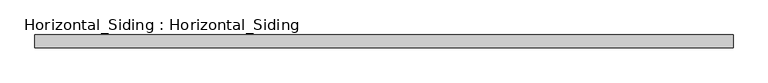
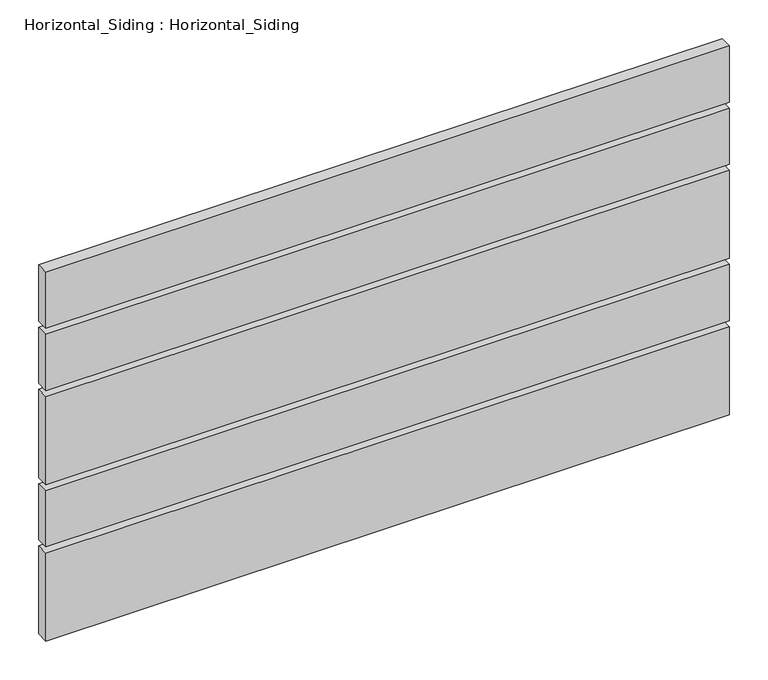
"""IFC4 building model written with IfcOpenShell, lengths in millimetres: plate geometry, Horizontal_Siding : Horizontal_Siding."""

from ifc_helpers import new_model, si_unit, frame, origin, place, context, project, spatial, polyline, outline, extrude, source, transform, mapped, element, save


def horizontal_siding_horizontal_siding_4d57135c(model_context):
    return source(origin(), model_context, "Body", "SweptSolid", [
        extrude(outline(polyline([(511.725524, -19.05), (-511.725524, -19.05), (-511.725524, 0.0), (511.725524, 0.0), (511.725524, -19.05)])), frame((0.0, 0.0, 9.525), z_axis=(0.0, 0.0, 1.0), x_axis=(1.0, 0.0, 0.0)), (0.0, 0.0, 1.0), 139.7),
        extrude(outline(polyline([(511.725524, -19.05), (-511.725524, -19.05), (-511.725524, 0.0), (511.725524, 0.0), (511.725524, -19.05)])), frame((0.0, 0.0, 158.75), z_axis=(0.0, 0.0, 1.0), x_axis=(1.0, 0.0, 0.0)), (0.0, 0.0, 1.0), 88.9),
        extrude(outline(polyline([(511.725524, -19.05), (-511.725524, -19.05), (-511.725524, 0.0), (511.725524, 0.0), (511.725524, -19.05)])), frame((0.0, 0.0, 257.175), z_axis=(0.0, 0.0, 1.0), x_axis=(1.0, 0.0, 0.0)), (0.0, 0.0, 1.0), 139.7),
        extrude(outline(polyline([(511.725524, -19.05), (-511.725524, -19.05), (-511.725524, 0.0), (511.725524, 0.0), (511.725524, -19.05)])), frame((0.0, 0.0, 406.4), z_axis=(0.0, 0.0, 1.0), x_axis=(1.0, 0.0, 0.0)), (0.0, 0.0, 1.0), 88.9),
        extrude(outline(polyline([(511.725524, -19.05), (-511.725524, -19.05), (-511.725524, 0.0), (511.725524, 0.0), (511.725524, -19.05)])), frame((0.0, 0.0, 504.825), z_axis=(0.0, 0.0, 1.0), x_axis=(1.0, 0.0, 0.0)), (0.0, 0.0, 1.0), 88.9),
    ])


if __name__ == "__main__":
    model = new_model("IFC4")
    model_context = context("Model", 3, world=origin())
    ifc_project = project(units=[si_unit("LENGTHUNIT", "METRE", prefix="MILLI")], contexts=[model_context])
    site = spatial("IfcSite", under=ifc_project)
    building = spatial("IfcBuilding", under=site)
    placement = place(None, origin())
    horizontal_siding_horizontal_siding_shape = horizontal_siding_horizontal_siding_4d57135c(model_context)
    element("IfcPlate", 1, ObjectType="Horizontal_Siding : Horizontal_Siding", at=placement, inside=building, context=model_context, shape_type="MappedRepresentation", body=[
        mapped(horizontal_siding_horizontal_siding_shape, transform((0.0, 0.0, 0.0), x_axis=(1.0, 0.0, 0.0), y_axis=(0.0, 1.0, 0.0), z_axis=(0.0, 0.0, 1.0))),
    ])
    save(model, "model.ifc")

# Revit data of these elements
# Type "Horizontal_Siding : Horizontal_Siding"
#   Analytic Construction = "<None>"
#   extend = 0' - 2 3/4"
#   Width_2 = 0' - 3 1/2"
#   Width_1 = 0' - 5 1/2"
#   Gap = 0' - 0 3/8"
#   Plank Material = SLOTTED WOOD FENCE (THERMALLY MODIFIED WOOD: ARBOR WOOD)\n(EXTERIOR STAIN : PENOFIN VERDE EXT. STAIN - COLOR: CEDAR)
# Element 1 (IfcPlate, "Horizontal_Siding : Horizontal_Siding")
#   Materials on its faces: "SLOTTED WOOD FENCE (THERMALLY MODIFIED WOOD: ARBOR WOOD)\n(EXTERIOR STAIN : PENOFIN VERDE EXT. STAIN - COLOR: CEDAR)"
# Materials
#   "SLOTTED WOOD FENCE (THERMALLY MODIFIED WOOD: ARBOR WOOD)\n(EXTERIOR STAIN : PENOFIN VERDE EXT. STAIN - COLOR: CEDAR)": class "Wood", colour RGB 164 134 123, transparency 0, Description = "Pinus Echinata", Cost = 0
